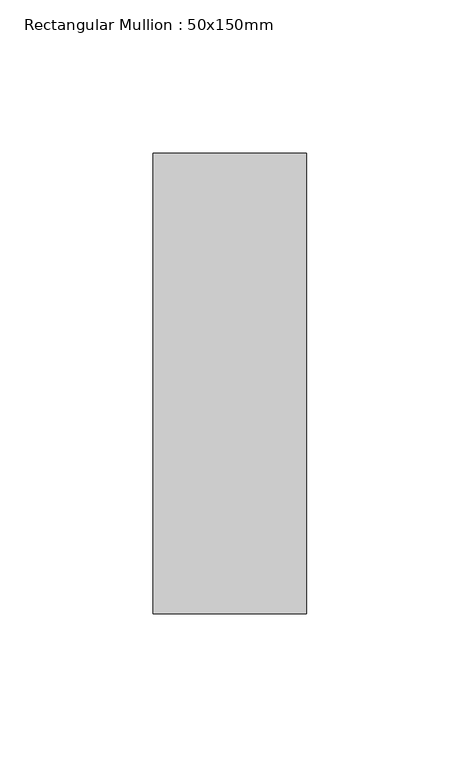
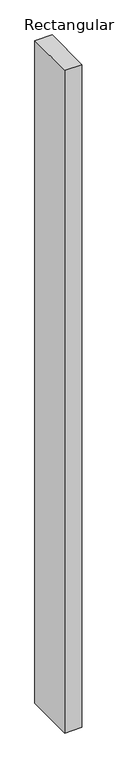
"""IFC4 building model written with IfcOpenShell, lengths in millimetres: member geometry, Rectangular Mullion : 50x150mm."""

from ifc_helpers import new_model, si_unit, frame, origin, place, context, project, spatial, polyline, outline, extrude, source, transform, mapped, element, save


def rectangular_mullion_50x150mm_ed10f38a(model_context):
    return source(origin(), model_context, "Body", "SweptSolid", [
        extrude(outline(polyline([(0.0, 75.0), (0.0, -75.0), (-50.0, -75.0), (-50.0, 75.0), (0.0, 75.0)])), frame((0.0, 0.0, -2034.1016494), z_axis=(0.0, 0.0, 1.0), x_axis=(1.0, 0.0, 0.0)), (0.0, 0.0, 1.0), 2034.1016494),
    ])


if __name__ == "__main__":
    model = new_model("IFC4")
    model_context = context("Model", 3, world=origin())
    ifc_project = project(units=[si_unit("LENGTHUNIT", "METRE", prefix="MILLI")], contexts=[model_context])
    site = spatial("IfcSite", under=ifc_project)
    building = spatial("IfcBuilding", under=site)
    placement = place(None, origin())
    rectangular_mullion_50x150mm_shape = rectangular_mullion_50x150mm_ed10f38a(model_context)
    element("IfcMember", 1, ObjectType="Rectangular Mullion : 50x150mm", at=placement, inside=building, context=model_context, shape_type="MappedRepresentation", body=[
        mapped(rectangular_mullion_50x150mm_shape, transform((0.0, 0.0, 0.0), x_axis=(1.0, 0.0, 0.0), y_axis=(0.0, 1.0, 0.0), z_axis=(0.0, 0.0, 1.0))),
    ])
    save(model, "model.ifc")

# Revit data of these elements
# Type "Rectangular Mullion : 50x150mm"
#   Keynote = "H11"
#   built-in parameter 1007304 = 0.492126 (stored number, unit not read)
#   built-in parameter 1007301 = 0.082021 (stored number, unit not read)
#   built-in parameter 1007300 = 0.082021 (stored number, unit not read)
# Element 1 (IfcMember, "Rectangular Mullion : 50x150mm")
#   Materials on its faces: "Aluminium"
# Materials
#   "Aluminium": class "Metal", colour RGB 247 247 247, transparency 0, Description = "Aluminium 6061", Cost = 0
